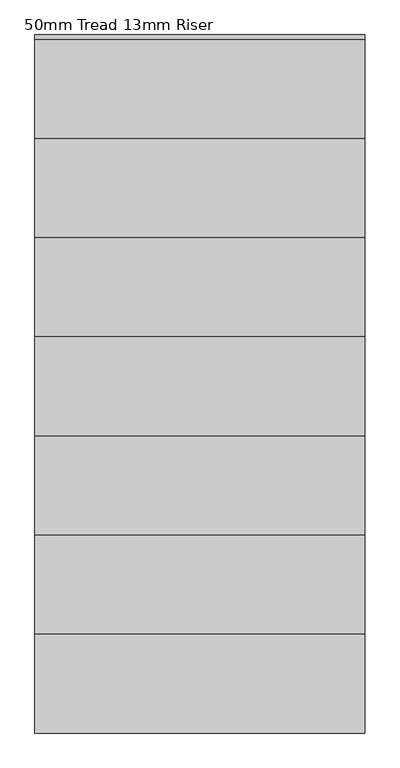
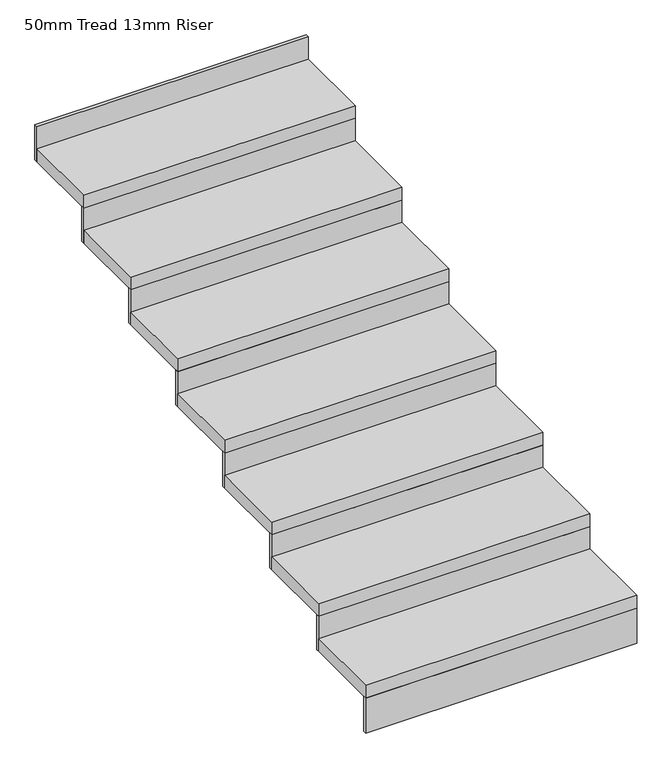
"""IFC4 building model written with IfcOpenShell, lengths in millimetres: stair flight geometry, 50mm Tread 13mm Riser."""

from ifc_helpers import new_model, si_unit, frame, origin, place, context, project, spatial, polyline, outline, extrude, source, transform, mapped, element, save


def stair_flight_50mm_tread_13mm_riser_7b211c03(model_context):
    return source(origin(), model_context, "Body", "SweptSolid", [
        extrude(outline(polyline([(22549.836337, -2888.024372), (22549.836337, -2900.524372), (21549.836337, -2900.524372), (21549.836337, -2888.024372), (22549.836337, -2888.024372)])), frame((0.0, 0.0, 1859.0909091), z_axis=(0.0, 0.0, 1.0), x_axis=(1.0, 0.0, 0.0)), (0.0, 0.0, 1.0), 136.3636364),
        extrude(outline(polyline([(21549.836337, -2600.524372), (22549.836337, -2600.524372), (22549.836337, -2900.524372), (21549.836337, -2900.524372), (21549.836337, -2600.524372)])), frame((0.0, 0.0, 1995.4545455), z_axis=(0.0, 0.0, 1.0), x_axis=(1.0, 0.0, 0.0)), (0.0, 0.0, 1.0), 50.0),
        extrude(outline(polyline([(22549.836337, -2588.024372), (22549.836337, -2600.524372), (21549.836337, -2600.524372), (21549.836337, -2588.024372), (22549.836337, -2588.024372)])), frame((0.0, 0.0, 1995.4545455), z_axis=(0.0, 0.0, 1.0), x_axis=(1.0, 0.0, 0.0)), (0.0, 0.0, 1.0), 136.3636364),
        extrude(outline(polyline([(21549.836337, -2300.524372), (22549.836337, -2300.524372), (22549.836337, -2600.524372), (21549.836337, -2600.524372), (21549.836337, -2300.524372)])), frame((0.0, 0.0, 2131.8181818), z_axis=(0.0, 0.0, 1.0), x_axis=(1.0, 0.0, 0.0)), (0.0, 0.0, 1.0), 50.0),
        extrude(outline(polyline([(22549.836337, -2288.024372), (22549.836337, -2300.524372), (21549.836337, -2300.524372), (21549.836337, -2288.024372), (22549.836337, -2288.024372)])), frame((0.0, 0.0, 2131.8181818), z_axis=(0.0, 0.0, 1.0), x_axis=(1.0, 0.0, 0.0)), (0.0, 0.0, 1.0), 136.3636364),
        extrude(outline(polyline([(21549.836337, -2000.524372), (22549.836337, -2000.524372), (22549.836337, -2300.524372), (21549.836337, -2300.524372), (21549.836337, -2000.524372)])), frame((0.0, 0.0, 2268.1818182), z_axis=(0.0, 0.0, 1.0), x_axis=(1.0, 0.0, 0.0)), (0.0, 0.0, 1.0), 50.0),
        extrude(outline(polyline([(22549.836337, -1988.024372), (22549.836337, -2000.524372), (21549.836337, -2000.524372), (21549.836337, -1988.024372), (22549.836337, -1988.024372)])), frame((0.0, 0.0, 2268.1818182), z_axis=(0.0, 0.0, 1.0), x_axis=(1.0, 0.0, 0.0)), (0.0, 0.0, 1.0), 136.3636364),
        extrude(outline(polyline([(21549.836337, -1700.524372), (22549.836337, -1700.524372), (22549.836337, -2000.524372), (21549.836337, -2000.524372), (21549.836337, -1700.524372)])), frame((0.0, 0.0, 2404.5454545), z_axis=(0.0, 0.0, 1.0), x_axis=(1.0, 0.0, 0.0)), (0.0, 0.0, 1.0), 50.0),
        extrude(outline(polyline([(22549.836337, -1688.024372), (22549.836337, -1700.524372), (21549.836337, -1700.524372), (21549.836337, -1688.024372), (22549.836337, -1688.024372)])), frame((0.0, 0.0, 2404.5454545), z_axis=(0.0, 0.0, 1.0), x_axis=(1.0, 0.0, 0.0)), (0.0, 0.0, 1.0), 136.3636364),
        extrude(outline(polyline([(21549.836337, -1400.524372), (22549.836337, -1400.524372), (22549.836337, -1700.524372), (21549.836337, -1700.524372), (21549.836337, -1400.524372)])), frame((0.0, 0.0, 2540.9090909), z_axis=(0.0, 0.0, 1.0), x_axis=(1.0, 0.0, 0.0)), (0.0, 0.0, 1.0), 50.0),
        extrude(outline(polyline([(22549.836337, -1388.024372), (22549.836337, -1400.524372), (21549.836337, -1400.524372), (21549.836337, -1388.024372), (22549.836337, -1388.024372)])), frame((0.0, 0.0, 2540.9090909), z_axis=(0.0, 0.0, 1.0), x_axis=(1.0, 0.0, 0.0)), (0.0, 0.0, 1.0), 136.3636364),
        extrude(outline(polyline([(21549.836337, -1100.524372), (22549.836337, -1100.524372), (22549.836337, -1400.524372), (21549.836337, -1400.524372), (21549.836337, -1100.524372)])), frame((0.0, 0.0, 2677.2727273), z_axis=(0.0, 0.0, 1.0), x_axis=(1.0, 0.0, 0.0)), (0.0, 0.0, 1.0), 50.0),
        extrude(outline(polyline([(22549.836337, -1088.024372), (22549.836337, -1100.524372), (21549.836337, -1100.524372), (21549.836337, -1088.024372), (22549.836337, -1088.024372)])), frame((0.0, 0.0, 2677.2727273), z_axis=(0.0, 0.0, 1.0), x_axis=(1.0, 0.0, 0.0)), (0.0, 0.0, 1.0), 136.3636364),
        extrude(outline(polyline([(21549.836337, -800.524372), (22549.836337, -800.524372), (22549.836337, -1100.524372), (21549.836337, -1100.524372), (21549.836337, -800.524372)])), frame((0.0, 0.0, 2813.6363636), z_axis=(0.0, 0.0, 1.0), x_axis=(1.0, 0.0, 0.0)), (0.0, 0.0, 1.0), 50.0),
        extrude(outline(polyline([(22549.836337, -788.024372), (22549.836337, -800.524372), (21549.836337, -800.524372), (21549.836337, -788.024372), (22549.836337, -788.024372)])), frame((0.0, 0.0, 2813.6363636), z_axis=(0.0, 0.0, 1.0), x_axis=(1.0, 0.0, 0.0)), (0.0, 0.0, 1.0), 136.3636364),
    ])


if __name__ == "__main__":
    model = new_model("IFC4")
    model_context = context("Model", 3, world=origin())
    ifc_project = project(units=[si_unit("LENGTHUNIT", "METRE", prefix="MILLI")], contexts=[model_context])
    site = spatial("IfcSite", under=ifc_project)
    building = spatial("IfcBuilding", under=site)
    placement = place(None, origin())
    stair_flight_50mm_tread_13mm_riser_shape = stair_flight_50mm_tread_13mm_riser_7b211c03(model_context)
    element("IfcStairFlight", 1, ObjectType="50mm Tread 13mm Riser", at=placement, inside=building, context=model_context, shape_type="MappedRepresentation", body=[
        mapped(stair_flight_50mm_tread_13mm_riser_shape, transform((0.0, 0.0, 0.0), x_axis=(1.0, 0.0, 0.0), y_axis=(0.0, 1.0, 0.0), z_axis=(0.0, 0.0, 1.0))),
    ])
    save(model, "model.ifc")
